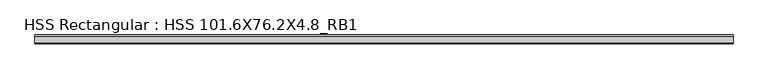
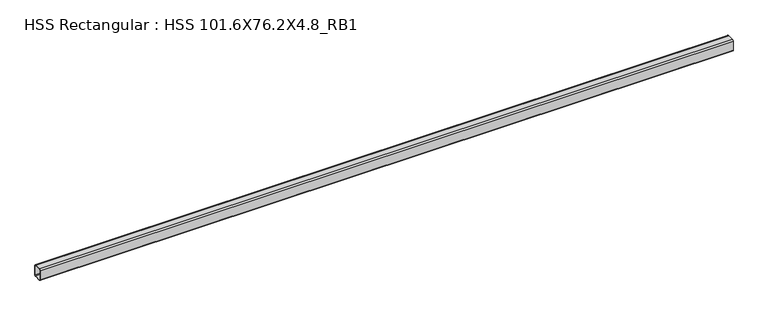
"""IFC4 building model written with IfcOpenShell, lengths in millimetres: beam geometry, HSS Rectangular : HSS 101.6X76.2X4.8_RB1."""

from ifc_helpers import new_model, si_unit, point, frame, frame_2d, origin, place, context, project, spatial, polyline, circle_curve, trimmed, segment, composite_curve, outline, extrude, source, transform, mapped, element, save


def hss_rectangular_hss_101_6x76_2x4_8_rb1_e40fc11b(model_context):
    return source(origin(), model_context, "Body", "SweptSolid", [
        extrude(outline(composite_curve([segment(polyline([(38.1, 41.275), (38.1, -41.275)]), True, "CONTINUOUS"), segment(trimmed(circle_curve(frame_2d((28.575, -41.275)), 9.525), [point((38.1, -41.275))], [point((28.575, -50.8))], False, "CARTESIAN"), True, "CONTINUOUS"), segment(polyline([(28.575, -50.8), (-28.575, -50.8)]), True, "CONTINUOUS"), segment(trimmed(circle_curve(frame_2d((-28.575, -41.275)), 9.525), [point((-28.575, -50.8))], [point((-38.1, -41.275))], False, "CARTESIAN"), True, "CONTINUOUS"), segment(polyline([(-38.1, -41.275), (-38.1, 41.275)]), True, "CONTINUOUS"), segment(trimmed(circle_curve(frame_2d((-28.575, 41.275)), 9.525), [point((-38.1, 41.275))], [point((-28.575, 50.8))], False, "CARTESIAN"), True, "CONTINUOUS"), segment(polyline([(-28.575, 50.8), (28.575, 50.8)]), True, "CONTINUOUS"), segment(trimmed(circle_curve(frame_2d((28.575, 41.275)), 9.525), [point((28.575, 50.8))], [point((38.1, 41.275))], False, "CARTESIAN"), True, "CONTINUOUS")], self_intersect=False), holes=[composite_curve([segment(trimmed(circle_curve(frame_2d((-28.575, 41.275)), 4.7625), [point((-28.575, 46.0375))], [point((-33.3375, 41.275))], True, "CARTESIAN"), True, "CONTINUOUS"), segment(polyline([(-33.3375, 41.275), (-33.3375, -41.275)]), True, "CONTINUOUS"), segment(trimmed(circle_curve(frame_2d((-28.575, -41.275)), 4.7625), [point((-33.3375, -41.275))], [point((-28.575, -46.0375))], True, "CARTESIAN"), True, "CONTINUOUS"), segment(polyline([(-28.575, -46.0375), (28.575, -46.0375)]), True, "CONTINUOUS"), segment(trimmed(circle_curve(frame_2d((28.575, -41.275)), 4.7625), [point((28.575, -46.0375))], [point((33.3375, -41.275))], True, "CARTESIAN"), True, "CONTINUOUS"), segment(polyline([(33.3375, -41.275), (33.3375, 41.275)]), True, "CONTINUOUS"), segment(trimmed(circle_curve(frame_2d((28.575, 41.275)), 4.7625), [point((33.3375, 41.275))], [point((28.575, 46.0375))], True, "CARTESIAN"), True, "CONTINUOUS"), segment(polyline([(28.575, 46.0375), (-28.575, 46.0375)]), True, "CONTINUOUS")], self_intersect=False)]), frame((1636.9347881, 0.0, 0.0), z_axis=(1.0, 0.0, 0.0), x_axis=(0.0, 1.0, 0.0)), (0.0, 0.0, 1.0), 5922.2898079),
    ])


if __name__ == "__main__":
    model = new_model("IFC4")
    model_context = context("Model", 3, world=origin())
    ifc_project = project(units=[si_unit("LENGTHUNIT", "METRE", prefix="MILLI")], contexts=[model_context])
    site = spatial("IfcSite", under=ifc_project)
    building = spatial("IfcBuilding", under=site)
    placement = place(None, origin())
    hss_rectangular_hss_101_6x76_2x4_8_rb1_shape = hss_rectangular_hss_101_6x76_2x4_8_rb1_e40fc11b(model_context)
    element("IfcBeam", 1, ObjectType="HSS Rectangular : HSS 101.6X76.2X4.8_RB1", at=placement, inside=building, context=model_context, shape_type="MappedRepresentation", body=[
        mapped(hss_rectangular_hss_101_6x76_2x4_8_rb1_shape, transform((0.0, 0.0, 0.0), x_axis=(1.0, 0.0, 0.0), y_axis=(0.0, 1.0, 0.0), z_axis=(0.0, 0.0, 1.0))),
    ])
    save(model, "model.ifc")

# Revit data of these elements
# Type "HSS Rectangular : HSS 101.6X76.2X4.8_RB1"
#   Section Name Key = "HSS 4X3X3/16"
#   Assembly Code = "B10"
#   Width = 7.62 cm
#   Wall Nominal Thickness = 0.4763 cm
#   Wall Design Thickness = 0.442 cm
#   Torsional Moment of Inertia = 260.561 cm⁴
#   Torsional Modulus = 61.2876 cm³
#   Section Area = 14.4516 cm²
#   Plastic Modulus weak axis = 40.3122 cm³
#   Plastic Modulus strong axis = 49.1612 cm³
#   Perimeter = 0.881482 m²/m
#   Outer Fillet = 0.9525 cm
#   Nominal Weight = 12.1285 kgf/m
#   Moment of Inertia weak axis = 131.529 cm⁴
#   Moment of Inertia strong axis = 205.202 cm⁴
#   Inner Fillet = 0.4763 cm
#   Height = 10.16 cm
#   Elastic Modulus weak axis = 34.4128 cm³
#   Elastic Modulus strong axis = 40.476 cm³
#   Centroid Vertical = 5.08 cm
#   Centroid Horizontal = 3.81 cm
#   Length [instance default] = 1524 mm
#   Structural Material [instance default] = Steel ASTM A500, Grade B, Rectangular and Square
#   Principal Axes Angle = 0
# Element 1 (IfcBeam, "HSS Rectangular : HSS 101.6X76.2X4.8_RB1")
#   Structural Material = Steel ASTM A992
#   Materials on its faces: "Steel ASTM A992"
# Materials
#   "Steel ASTM A500, Grade B, Rectangular and Square": class "Metal", colour RGB 199 199 199, transparency 0, Description = "Carbon steel", Cost = 0
#   "Steel ASTM A992": class "Metal", colour RGB 199 199 199, transparency 0, Description = "Structural steel 50ksi", Cost = 0
